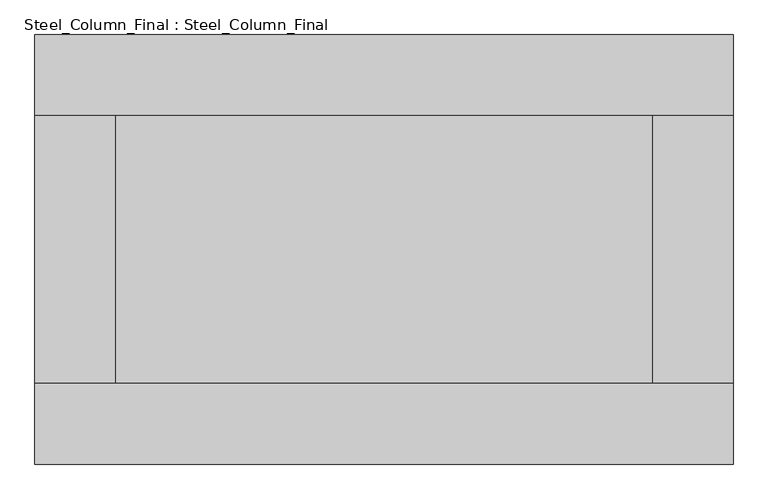
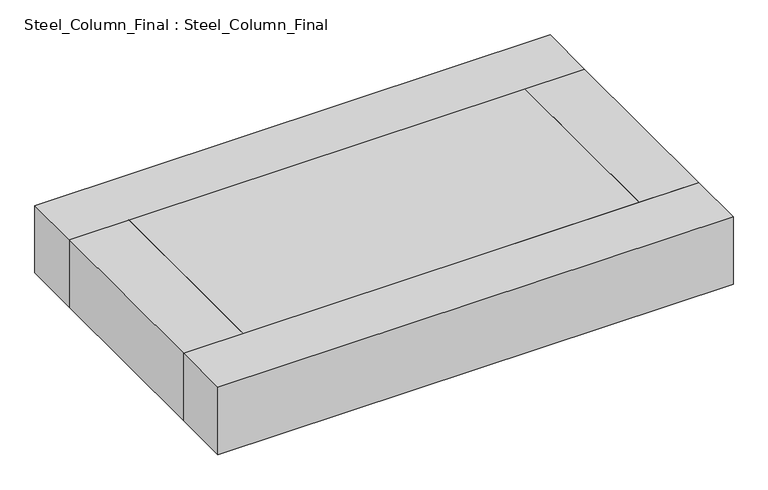
"""IFC4 building model written with IfcOpenShell, lengths in millimetres: proxy geometry, Steel_Column_Final : Steel_Column_Final."""

from ifc_helpers import new_model, si_unit, frame, origin, place, context, project, spatial, polyline, outline, extrude, source, transform, mapped, element, save


def steel_column_final_steel_column_final_0e6d6ca0(model_context):
    return source(origin(), model_context, "Body", "SweptSolid", [
        extrude(outline(polyline([(6500.0, 2500.0), (-6500.0, 2500.0), (-6500.0, 4000.0), (6500.0, 4000.0), (6500.0, 2500.0)])), frame((0.0, 0.0, 14194.0), z_axis=(0.0, 0.0, 1.0), x_axis=(1.0, 0.0, 0.0)), (0.0, 0.0, 1.0), 1800.0),
        extrude(outline(polyline([(-6500.0, -2500.0), (6500.0, -2500.0), (6500.0, -4000.0), (-6500.0, -4000.0), (-6500.0, -2500.0)])), frame((0.0, 0.0, 14194.0), z_axis=(0.0, 0.0, 1.0), x_axis=(1.0, 0.0, 0.0)), (0.0, 0.0, 1.0), 1800.0),
        extrude(outline(polyline([(5000.0, -2500.0), (5000.0, 2500.0), (6500.0, 2500.0), (6500.0, -2500.0), (5000.0, -2500.0)])), frame((0.0, 0.0, 14194.0), z_axis=(0.0, 0.0, 1.0), x_axis=(1.0, 0.0, 0.0)), (0.0, 0.0, 1.0), 1800.0),
        extrude(outline(polyline([(-5000.0, 2500.0), (-5000.0, -2500.0), (-6500.0, -2500.0), (-6500.0, 2500.0), (-5000.0, 2500.0)])), frame((0.0, 0.0, 14194.0), z_axis=(0.0, 0.0, 1.0), x_axis=(1.0, 0.0, 0.0)), (0.0, 0.0, 1.0), 1800.0),
        extrude(outline(polyline([(-5000.0, -2500.0), (-5000.0, 2500.0), (5000.0, 2500.0), (5000.0, -2500.0), (-5000.0, -2500.0)])), frame((0.0, 0.0, 14194.0), z_axis=(0.0, 0.0, 1.0), x_axis=(1.0, 0.0, 0.0)), (0.0, 0.0, 1.0), 1800.0),
    ])


if __name__ == "__main__":
    model = new_model("IFC4")
    model_context = context("Model", 3, world=origin())
    ifc_project = project(units=[si_unit("LENGTHUNIT", "METRE", prefix="MILLI")], contexts=[model_context])
    site = spatial("IfcSite", under=ifc_project)
    building = spatial("IfcBuilding", under=site)
    placement = place(None, origin())
    steel_column_final_steel_column_final_shape = steel_column_final_steel_column_final_0e6d6ca0(model_context)
    element("IfcBuildingElementProxy", 1, Name="Steel_Column_Final : Steel_Column_Final", ObjectType="Steel_Column_Final : Steel_Column_Final", at=placement, inside=building, context=model_context, shape_type="MappedRepresentation", body=[
        mapped(steel_column_final_steel_column_final_shape, transform((0.0, 0.0, 0.0), x_axis=(1.0, 0.0, 0.0), y_axis=(0.0, 1.0, 0.0), z_axis=(0.0, 0.0, 1.0))),
    ])
    save(model, "model.ifc")

# Revit data of these elements
# Type "Steel_Column_Final : Steel_Column_Final"
#   Top Width [instance default] = 5000 mm
#   Top Length = 10000 mm
#   Length = 21000 mm
#   Height [instance default] = 50000 mm
#   Bottom Width [instance default] = 5000 mm
#   Default Elevation = 0
# Element 1 (IfcBuildingElementProxy, "Steel_Column_Final : Steel_Column_Final")
#   Height = 14194 mm
